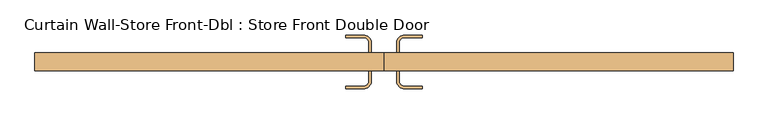
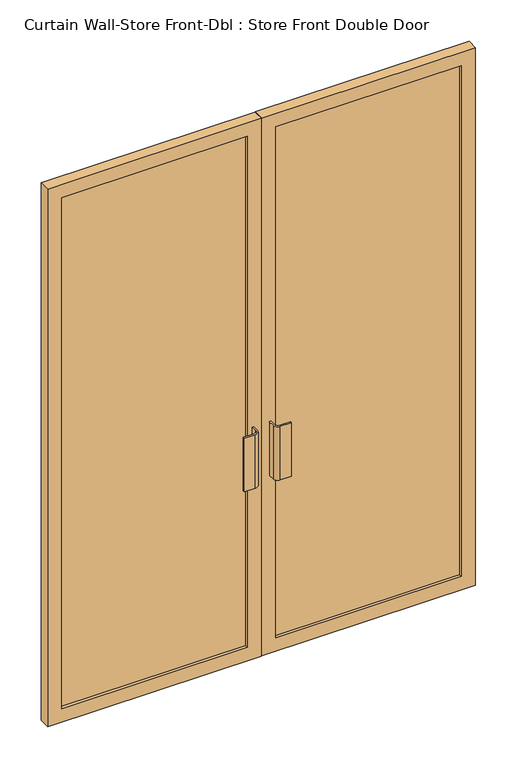
"""IFC4 building model written with IfcOpenShell, lengths in millimetres: door geometry, Curtain Wall-Store Front-Dbl : Store Front Double Door."""

from ifc_helpers import new_model, si_unit, point, frame, frame_2d, origin, place, context, project, spatial, polyline, circle_curve, trimmed, segment, composite_curve, outline, extrude, source, transform, mapped, element, save


def curtain_wall_store_front_dbl_store_front_double_door_239a7903(model_context):
    return source(origin(), model_context, "Body", "SweptSolid", [
        extrude(outline(composite_curve([segment(polyline([(-31.75, 12.7), (-31.75, -12.7), (-38.1, -12.7), (-38.1, 12.7)]), True, "CONTINUOUS"), segment(trimmed(circle_curve(frame_2d((-50.8, 12.7)), 12.7), [point((-38.1, 12.7))], [point((-50.8, 25.4))], True, "CARTESIAN"), True, "CONTINUOUS"), segment(polyline([(-50.8, 25.4), (-95.25, 25.4), (-95.25, 31.75), (-50.8, 31.75)]), True, "CONTINUOUS"), segment(trimmed(circle_curve(frame_2d((-50.8, 12.7)), 19.05), [point((-50.8, 31.75))], [point((-31.75, 12.7))], False, "CARTESIAN"), True, "CONTINUOUS")], self_intersect=False)), frame((0.0, 0.0, 762.0), z_axis=(0.0, 0.0, 1.0), x_axis=(1.0, 0.0, 0.0)), (0.0, 0.0, 1.0), 228.6),
        extrude(outline(composite_curve([segment(trimmed(circle_curve(frame_2d((50.8, 12.7)), 19.05), [point((31.75, 12.7))], [point((50.8, 31.75))], False, "CARTESIAN"), True, "CONTINUOUS"), segment(polyline([(50.8, 31.75), (95.25, 31.75), (95.25, 25.4), (50.8, 25.4)]), True, "CONTINUOUS"), segment(trimmed(circle_curve(frame_2d((50.8, 12.7)), 12.7), [point((50.8, 25.4))], [point((38.1, 12.7))], True, "CARTESIAN"), True, "CONTINUOUS"), segment(polyline([(38.1, 12.7), (38.1, -12.7), (31.75, -12.7), (31.75, 12.7)]), True, "CONTINUOUS")], self_intersect=False)), frame((0.0, 0.0, 762.0), z_axis=(0.0, 0.0, 1.0), x_axis=(1.0, 0.0, 0.0)), (0.0, 0.0, 1.0), 228.6),
        extrude(outline(composite_curve([segment(trimmed(circle_curve(frame_2d((-50.8, -82.55)), 19.05), [point((-31.75, -82.55))], [point((-50.8, -101.6))], False, "CARTESIAN"), True, "CONTINUOUS"), segment(polyline([(-50.8, -101.6), (-95.25, -101.6), (-95.25, -95.25), (-50.8, -95.25)]), True, "CONTINUOUS"), segment(trimmed(circle_curve(frame_2d((-50.8, -82.55)), 12.7), [point((-50.8, -95.25))], [point((-38.1, -82.55))], True, "CARTESIAN"), True, "CONTINUOUS"), segment(polyline([(-38.1, -82.55), (-38.1, -57.15), (-31.75, -57.15), (-31.75, -82.55)]), True, "CONTINUOUS")], self_intersect=False)), frame((0.0, 0.0, 762.0), z_axis=(0.0, 0.0, 1.0), x_axis=(1.0, 0.0, 0.0)), (0.0, 0.0, 1.0), 228.6),
        extrude(outline(composite_curve([segment(polyline([(31.75, -82.55), (31.75, -57.15), (38.1, -57.15), (38.1, -82.55)]), True, "CONTINUOUS"), segment(trimmed(circle_curve(frame_2d((50.8, -82.55)), 12.7), [point((38.1, -82.55))], [point((50.8, -95.25))], True, "CARTESIAN"), True, "CONTINUOUS"), segment(polyline([(50.8, -95.25), (95.25, -95.25), (95.25, -101.6), (50.8, -101.6)]), True, "CONTINUOUS"), segment(trimmed(circle_curve(frame_2d((50.8, -82.55)), 19.05), [point((50.8, -101.6))], [point((31.75, -82.55))], False, "CARTESIAN"), True, "CONTINUOUS")], self_intersect=False)), frame((0.0, 0.0, 762.0), z_axis=(0.0, 0.0, 1.0), x_axis=(1.0, 0.0, 0.0)), (0.0, 0.0, 1.0), 228.6),
        extrude(outline(polyline([(807.4671284, -25.4), (807.4671284, -44.45), (57.94375, -44.45), (57.94375, -25.4), (807.4671284, -25.4)])), frame((0.0, 0.0, 57.15), z_axis=(0.0, 0.0, 1.0), x_axis=(1.0, 0.0, 0.0)), (0.0, 0.0, 1.0), 2182.8125),
        extrude(outline(polyline([(-57.94375, -25.4), (-57.94375, -44.45), (-807.4671284, -44.45), (-807.4671284, -25.4), (-57.94375, -25.4)])), frame((0.0, 0.0, 57.15), z_axis=(0.0, 0.0, 1.0), x_axis=(1.0, 0.0, 0.0)), (0.0, 0.0, 1.0), 2182.8125),
        extrude(outline(polyline([(2297.1125, 0.79375), (0.0, 0.79375), (0.0, 864.6171284), (2297.1125, 864.6171284), (2297.1125, 0.79375)]), holes=[polyline([(2239.9625, 57.94375), (2239.9625, 807.4671284), (57.15, 807.4671284), (57.15, 57.94375), (2239.9625, 57.94375)])]), frame((0.0, -57.15, 0.0), z_axis=(0.0, 1.0, 0.0), x_axis=(0.0, 0.0, 1.0)), (0.0, 0.0, 1.0), 44.45),
        extrude(outline(polyline([(2297.1125, -0.79375), (2297.1125, -864.6171284), (0.0, -864.6171284), (0.0, -0.79375), (2297.1125, -0.79375)]), holes=[polyline([(2239.9625, -807.4671284), (2239.9625, -57.94375), (57.15, -57.94375), (57.15, -807.4671284), (2239.9625, -807.4671284)])]), frame((0.0, -57.15, 0.0), z_axis=(0.0, 1.0, 0.0), x_axis=(0.0, 0.0, 1.0)), (0.0, 0.0, 1.0), 44.45),
    ])


if __name__ == "__main__":
    model = new_model("IFC4")
    model_context = context("Model", 3, world=origin())
    ifc_project = project(units=[si_unit("LENGTHUNIT", "METRE", prefix="MILLI")], contexts=[model_context])
    site = spatial("IfcSite", under=ifc_project)
    building = spatial("IfcBuilding", under=site)
    placement = place(None, origin())
    curtain_wall_store_front_dbl_store_front_double_door_shape = curtain_wall_store_front_dbl_store_front_double_door_239a7903(model_context)
    element("IfcDoor", 1, ObjectType="Curtain Wall-Store Front-Dbl : Store Front Double Door", at=placement, inside=building, context=model_context, shape_type="MappedRepresentation", body=[
        mapped(curtain_wall_store_front_dbl_store_front_double_door_shape, transform((0.0, 0.0, 0.0), x_axis=(1.0, 0.0, 0.0), y_axis=(0.0, 1.0, 0.0), z_axis=(0.0, 0.0, 1.0))),
    ])
    save(model, "model.ifc")

# Revit data of these elements
# Type "Curtain Wall-Store Front-Dbl : Store Front Double Door"
#   Type Mark = "17"
#   Construction Type Id = "MDOOR"
#   Assembly Code = "B2030110"
#   Analytic Construction = "Metal"
#   Offset = 0' - 2 1/4"
#   Heat Transfer Coefficient (U) = 3.7021 W/(m²·K)
#   Function = 1
#   Material = Aluminum
#   Glazing Material = Glass
#   Visual Light Transmittance = 0
#   Solar Heat Gain Coefficient = 0
# Element 1 (IfcDoor, "Curtain Wall-Store Front-Dbl : Store Front Double Door")
#   Materials on its faces: "Aluminum", "Glass"
# Materials
#   "Aluminum": class "Metal", colour RGB 247 247 247, transparency 0, Description = "Aluminum 6061", Cost = 0
#   "Glass": class "Unassigned", colour RGB 0 0 255, transparency 0.75
